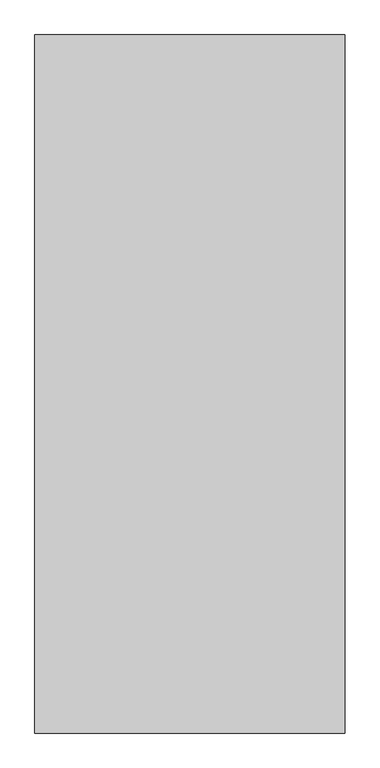
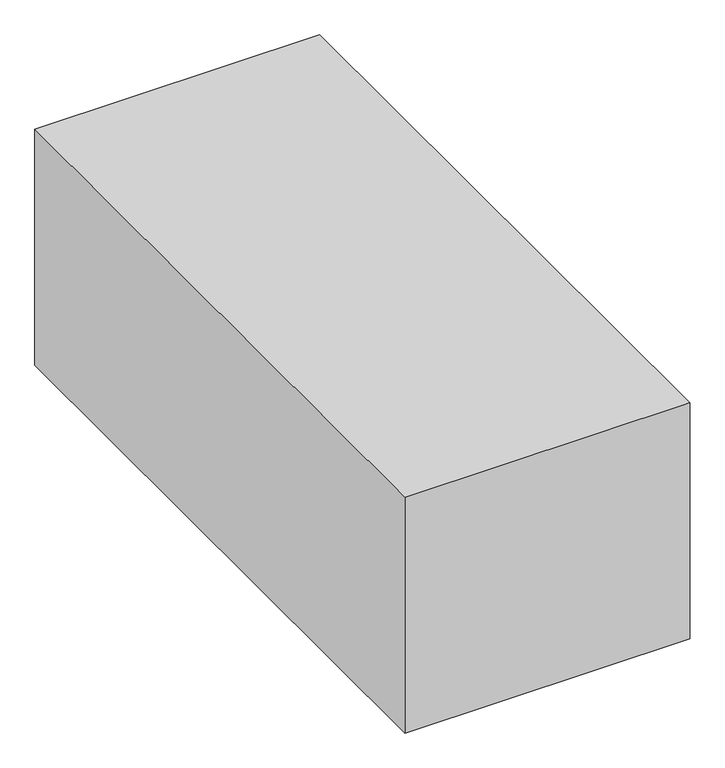
"""IFC4 building model written with IfcOpenShell, lengths in millimetres: proxy geometry, Space Planning Box_hec : Space Planning Box_hec."""

from ifc_helpers import new_model, si_unit, origin, origin_with_axes, place, context, project, spatial, polyline, outline, extrude, source, transform, mapped, element, save


def generic_models_0b067365(model_context):
    return source(origin(), model_context, "Body", "SweptSolid", [
        extrude(outline(polyline([(2000.0, 4500.0), (2000.0, -4500.0), (-2000.0, -4500.0), (-2000.0, 4500.0), (2000.0, 4500.0)])), origin_with_axes(), (0.0, 0.0, 1.0), 3500.0),
    ])


if __name__ == "__main__":
    model = new_model("IFC4")
    model_context = context("Model", 3, world=origin())
    ifc_project = project(units=[si_unit("LENGTHUNIT", "METRE", prefix="MILLI")], contexts=[model_context])
    site = spatial("IfcSite", under=ifc_project)
    building = spatial("IfcBuilding", under=site)
    placement = place(None, origin())
    generic_models_shape = generic_models_0b067365(model_context)
    element("IfcBuildingElementProxy", 1, Name="Space Planning Box_hec : Space Planning Box_hec", ObjectType="Space Planning Box_hec : Space Planning Box_hec", at=placement, inside=building, context=model_context, shape_type="MappedRepresentation", body=[
        mapped(generic_models_shape, transform((0.0, 0.0, 0.0), x_axis=(1.0, 0.0, 0.0), y_axis=(0.0, 1.0, 0.0), z_axis=(0.0, 0.0, 1.0))),
    ])
    save(model, "model.ifc")

# Revit data of these elements
# Type "Space Planning Box_hec : Space Planning Box_hec"
#   Type Comments = "..."
#   Room Name [instance default] = "?"
#   Interior Finish [instance default] = ""
#   Exterior Finish [instance default] = ""
#   Department [instance default] = ""
#   Assembly Code = "..."
#   ceiling height [instance default] = 0
#   Width [instance default] = 1524 mm
#   Program Area [instance default] = 0.00 m²
#   Length [instance default] = 1524 mm
#   Height [instance default] = 1524 mm
#   Area [instance default] = 2.32258 m²
#   Fill Color [instance default] = Cyan
#   Default Elevation = 0
# Element 1 (IfcBuildingElementProxy, "Space Planning Box_hec : Space Planning Box_hec")
#   Room Name = "Lobby"
#   Exterior Finish = "N/A..N/A,,EW2..N/A..N/A"
#   Department = "AR"
#   Width = 4000 mm
#   Length = 9000 mm
#   Height = 3500 mm
#   Area = 36.00 m²
#   Materials on its faces: "Cyan"
# Materials
#   "Cyan": class "Generic", colour RGB 0 255 255, transparency 0.2, Cost = 0
